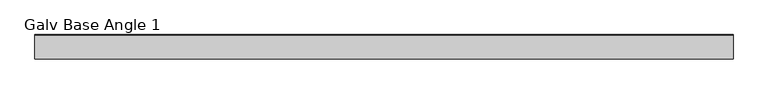
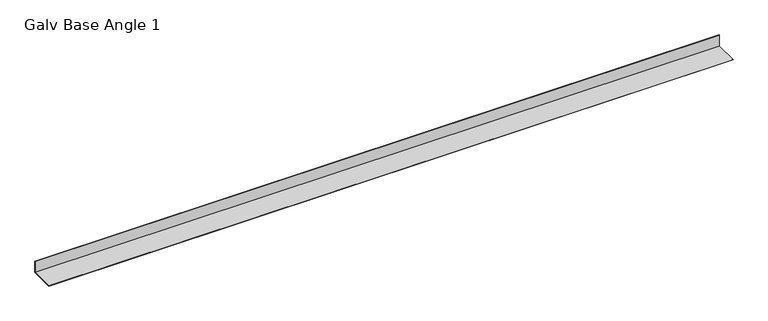
"""IFC4 building model written with IfcOpenShell, lengths in millimetres: proxy geometry, Galv Base Angle 1 : CF Galv L 4x2x16ga."""

from ifc_helpers import new_model, si_unit, frame, origin, place, context, project, spatial, polyline, outline, extrude, source, transform, mapped, element, save


def galv_base_angle_1_bf8ff121(model_context):
    return source(origin(), model_context, "Body", "SweptSolid", [
        extrude(outline(polyline([(-531741.6101341, 0.93726), (-531640.9473941, 0.93726), (-531640.9473941, 50.8), (-531640.0101341, 50.8), (-531640.0101341, 0.0), (-531741.6101341, 0.0), (-531741.6101341, 0.93726)])), frame((587411.9309739, 0.0, 0.0), z_axis=(1.0, 0.0, 0.0), x_axis=(0.0, 1.0, 0.0)), (0.0, 0.0, 1.0), 2906.7125),
    ])


if __name__ == "__main__":
    model = new_model("IFC4")
    model_context = context("Model", 3, world=origin())
    ifc_project = project(units=[si_unit("LENGTHUNIT", "METRE", prefix="MILLI")], contexts=[model_context])
    site = spatial("IfcSite", under=ifc_project)
    building = spatial("IfcBuilding", under=site)
    placement = place(None, origin())
    galv_base_angle_1_shape = galv_base_angle_1_bf8ff121(model_context)
    element("IfcBuildingElementProxy", 1, Name="Galv Base Angle 1 : CF Galv L 4x2x16ga", ObjectType="Galv Base Angle 1 : CF Galv L 4x2x16ga", at=placement, inside=building, context=model_context, shape_type="MappedRepresentation", body=[
        mapped(galv_base_angle_1_shape, transform((0.0, 0.0, 0.0), x_axis=(1.0, 0.0, 0.0), y_axis=(0.0, 1.0, 0.0), z_axis=(0.0, 0.0, 1.0))),
    ])
    save(model, "model.ifc")

# Revit data of these elements
# Element 1 (IfcBuildingElementProxy, "Galv Base Angle 1 : CF Galv L 4x2x16ga")
#   Materials on its faces: "4\"X2\" L - COLD-FORMED GALV."
# Materials
#   "4\"X2\" L - COLD-FORMED GALV.": class "Generic", colour RGB 143 142 141, transparency 0, Cost = 0
